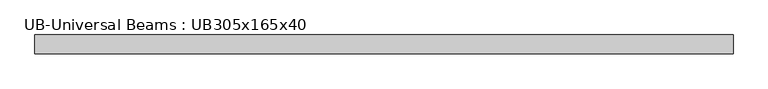
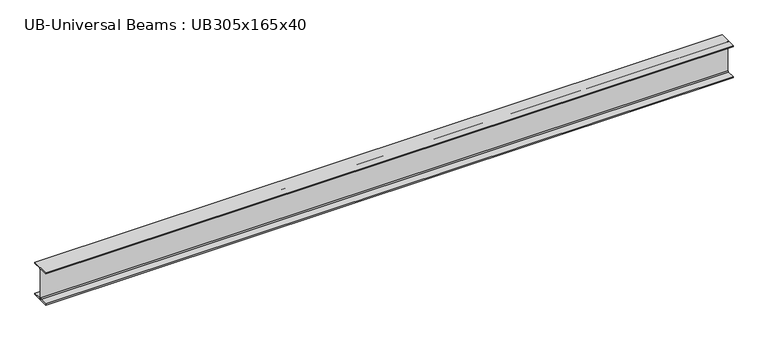
"""IFC4 building model written with IfcOpenShell, lengths in millimetres: beam geometry, UB-Universal Beams : UB305x165x40."""

from ifc_helpers import new_model, si_unit, point, frame, frame_2d, origin, place, context, project, spatial, polyline, circle_curve, trimmed, segment, composite_curve, outline, extrude, source, transform, mapped, element, save


def ub_universal_beams_ub305x165x40_ed37dae5(model_context):
    return source(origin(), model_context, "Body", "SweptSolid", [
        extrude(outline(composite_curve([segment(polyline([(82.5, -141.5), (82.5, -151.7), (-82.5, -151.7), (-82.5, -141.5), (-11.9, -141.5)]), True, "CONTINUOUS"), segment(trimmed(circle_curve(frame_2d((-11.9, -132.6)), 8.9), [point((-11.9, -141.5))], [point((-3.0, -132.6))], True, "CARTESIAN"), True, "CONTINUOUS"), segment(polyline([(-3.0, -132.6), (-3.0, 132.6)]), True, "CONTINUOUS"), segment(trimmed(circle_curve(frame_2d((-11.9, 132.6)), 8.9), [point((-3.0, 132.6))], [point((-11.9, 141.5))], True, "CARTESIAN"), True, "CONTINUOUS"), segment(polyline([(-11.9, 141.5), (-82.5, 141.5), (-82.5, 151.7), (82.5, 151.7), (82.5, 141.5), (11.9, 141.5)]), True, "CONTINUOUS"), segment(trimmed(circle_curve(frame_2d((11.9, 132.6)), 8.9), [point((11.9, 141.5))], [point((3.0, 132.6))], True, "CARTESIAN"), True, "CONTINUOUS"), segment(polyline([(3.0, 132.6), (3.0, -132.6)]), True, "CONTINUOUS"), segment(trimmed(circle_curve(frame_2d((11.9, -132.6)), 8.9), [point((3.0, -132.6))], [point((11.9, -141.5))], True, "CARTESIAN"), True, "CONTINUOUS"), segment(polyline([(11.9, -141.5), (82.5, -141.5)]), True, "CONTINUOUS")], self_intersect=False)), frame((-3051.6, 0.0, 0.0), z_axis=(1.0, 0.0, 0.0), x_axis=(0.0, 1.0, 0.0)), (0.0, 0.0, 1.0), 6103.2),
    ])


if __name__ == "__main__":
    model = new_model("IFC4")
    model_context = context("Model", 3, world=origin())
    ifc_project = project(units=[si_unit("LENGTHUNIT", "METRE", prefix="MILLI")], contexts=[model_context])
    site = spatial("IfcSite", under=ifc_project)
    building = spatial("IfcBuilding", under=site)
    placement = place(None, origin())
    ub_universal_beams_ub305x165x40_shape = ub_universal_beams_ub305x165x40_ed37dae5(model_context)
    element("IfcBeam", 1, ObjectType="UB-Universal Beams : UB305x165x40", at=placement, inside=building, context=model_context, shape_type="MappedRepresentation", body=[
        mapped(ub_universal_beams_ub305x165x40_shape, transform((0.0, 0.0, 0.0), x_axis=(1.0, 0.0, 0.0), y_axis=(0.0, 1.0, 0.0), z_axis=(0.0, 0.0, 1.0))),
    ])
    save(model, "model.ifc")

# Revit data of these elements
# Type "UB-Universal Beams : UB305x165x40"
#   Section Name Key = "UB305X165X40"
#   Width = 16.5 cm
#   Web Thickness = 0.6 cm
#   Web Fillet = 0.89 cm
#   Warping Constant = 164000.0 cm⁶
#   Torsional Moment of Inertia = 14.70 cm⁴
#   Section Area = 51.3 cm²
#   Plastic Modulus weak axis = 142.0 cm³
#   Plastic Modulus strong axis = 623.0 cm³
#   Nominal Weight = 40.2999 kgf/m
#   Moment of Inertia weak axis = 764.00 cm⁴
#   Moment of Inertia strong axis = 8503.00 cm⁴
#   Height = 30.34 cm
#   Flange Thickness = 1.02 cm
#   Elastic Modulus weak axis = 92.6 cm³
#   Elastic Modulus strong axis = 560.0 cm³
#   Centroid Vertical = 15.17 cm
#   Centroid Horizontal = 8.25 cm
#   Bolt Spacing = 9.0 cm
#   Length [instance default] = 1500 mm
#   Structural Material [instance default] = Metal - Steel 43-275
#   Type Comments = ""
#   Assembly Code = ""
# Element 1 (IfcBeam, "UB-Universal Beams : UB305x165x40")
#   Materials on its faces: "Metal - Steel 43-275"
# Materials
#   "Metal - Steel 43-275": class "Metal", colour RGB 247 247 247, transparency 0, Cost = 0
